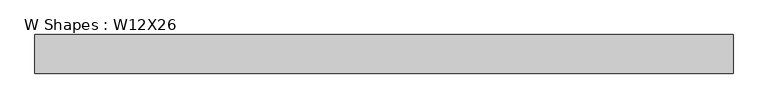
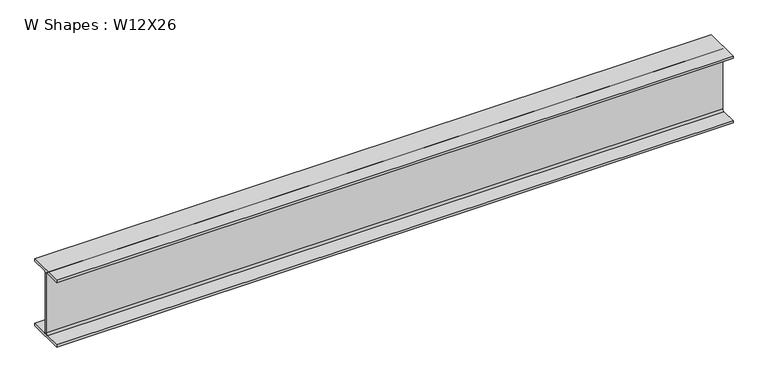
"""IFC4 building model written with IfcOpenShell, lengths in millimetres: beam geometry, W Shapes : W12X26."""

from ifc_helpers import new_model, si_unit, point, frame, frame_2d, origin, place, context, project, spatial, polyline, circle_curve, trimmed, segment, composite_curve, outline, extrude, source, transform, mapped, element, save


def w_shapes_w12x26_f5a50409(model_context):
    return source(origin(), model_context, "Body", "SweptSolid", [
        extrude(outline(composite_curve([segment(polyline([(82.423, -145.288), (82.423, -154.94), (-82.423, -154.94), (-82.423, -145.288), (-10.541, -145.288)]), True, "CONTINUOUS"), segment(trimmed(circle_curve(frame_2d((-10.541, -137.668)), 7.62), [point((-10.541, -145.288))], [point((-2.921, -137.668))], True, "CARTESIAN"), True, "CONTINUOUS"), segment(polyline([(-2.921, -137.668), (-2.921, 137.668)]), True, "CONTINUOUS"), segment(trimmed(circle_curve(frame_2d((-10.541, 137.668)), 7.62), [point((-2.921, 137.668))], [point((-10.541, 145.288))], True, "CARTESIAN"), True, "CONTINUOUS"), segment(polyline([(-10.541, 145.288), (-82.423, 145.288), (-82.423, 154.94), (82.423, 154.94), (82.423, 145.288), (10.541, 145.288)]), True, "CONTINUOUS"), segment(trimmed(circle_curve(frame_2d((10.541, 137.668)), 7.62), [point((10.541, 145.288))], [point((2.921, 137.668))], True, "CARTESIAN"), True, "CONTINUOUS"), segment(polyline([(2.921, 137.668), (2.921, -137.668)]), True, "CONTINUOUS"), segment(trimmed(circle_curve(frame_2d((10.541, -137.668)), 7.62), [point((2.921, -137.668))], [point((10.541, -145.288))], True, "CARTESIAN"), True, "CONTINUOUS"), segment(polyline([(10.541, -145.288), (82.423, -145.288)]), True, "CONTINUOUS")], self_intersect=False)), frame((-1498.6, 0.0, 0.0), z_axis=(1.0, 0.0, 0.0), x_axis=(0.0, 1.0, 0.0)), (0.0, 0.0, 1.0), 2978.15),
    ])


if __name__ == "__main__":
    model = new_model("IFC4")
    model_context = context("Model", 3, world=origin())
    ifc_project = project(units=[si_unit("LENGTHUNIT", "METRE", prefix="MILLI")], contexts=[model_context])
    site = spatial("IfcSite", under=ifc_project)
    building = spatial("IfcBuilding", under=site)
    placement = place(None, origin())
    w_shapes_w12x26_shape = w_shapes_w12x26_f5a50409(model_context)
    element("IfcBeam", 1, ObjectType="W Shapes : W12X26", at=placement, inside=building, context=model_context, shape_type="MappedRepresentation", body=[
        mapped(w_shapes_w12x26_shape, transform((0.0, 0.0, 0.0), x_axis=(1.0, 0.0, 0.0), y_axis=(0.0, 1.0, 0.0), z_axis=(0.0, 0.0, 1.0))),
    ])
    save(model, "model.ifc")

# Revit data of these elements
# Type "W Shapes : W12X26"
#   Section Name Key = "W12x26"
#   Assembly Code = "B10"
#   Width = 6.490"
#   Web Thickness = 0.230"
#   Web Fillet = 0.300"
#   Warping Constant = 607.00 in⁶
#   Torsional Moment of Inertia = 0.30 in⁴
#   Section Area = 7.65 in²
#   Plastic Modulus weak axis = 8.17 in³
#   Plastic Modulus strong axis = 37.20 in³
#   Perimeter = 4.12 ft²/ft
#   Nominal Weight = 26.00 lbf/ft
#   Moment of Inertia weak axis = 17.30 in⁴
#   Moment of Inertia strong axis = 204.00 in⁴
#   Height = 12.200"
#   Flange Thickness = 0.380"
#   Elastic Modulus weak axis = 5.34 in³
#   Elastic Modulus strong axis = 33.40 in³
#   Centroid Vertical = 6.100"
#   Centroid Horizontal = 3.245"
#   Bolt Spacing = 0' - 3 1/2"
#   Length [instance default] = 5' - 0"
#   Structural Material [instance default] = Steel ASTM A992
#   Principal Axes Angle = 0
# Element 1 (IfcBeam, "W Shapes : W12X26")
#   Materials on its faces: "Steel ASTM A992"
# Materials
#   "Steel ASTM A992": class "Metal", colour RGB 199 199 199, transparency 0, Description = "Structural steel 50ksi", Cost = 0
